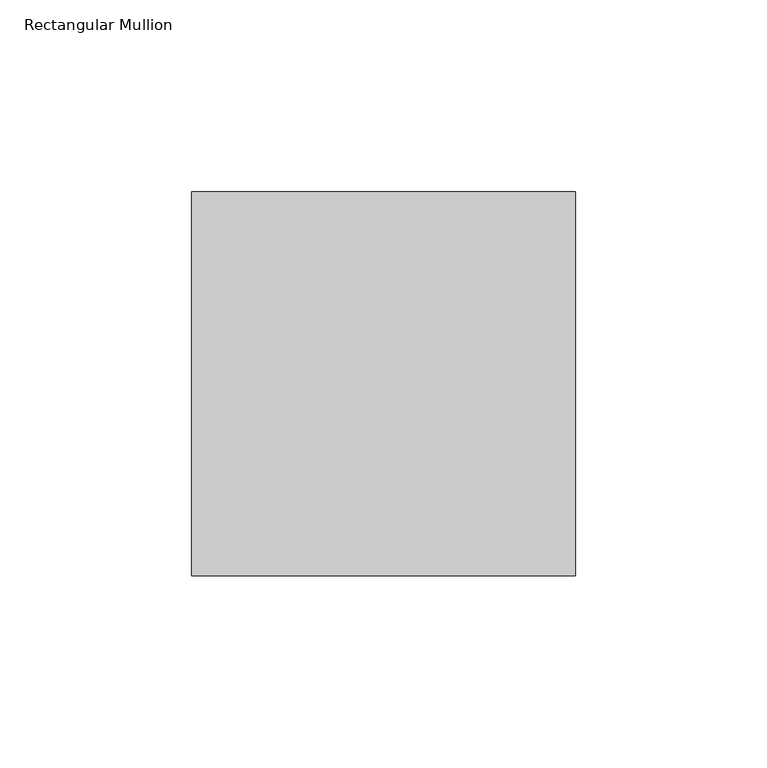
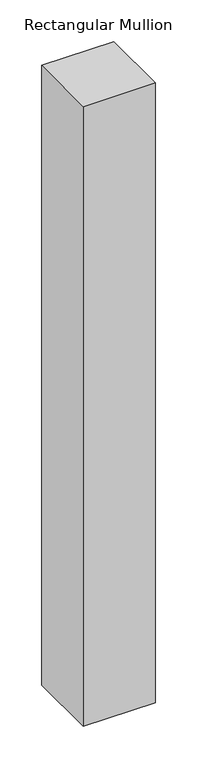
"""IFC4 building model written with IfcOpenShell, lengths in millimetres: member geometry, Rectangular Mullion : 알루미늄_Rectangular Cap_100 x100."""

from ifc_helpers import new_model, si_unit, frame, origin, place, context, project, spatial, polyline, outline, extrude, source, transform, mapped, element, save


def rectangular_mullion_dadccf76(model_context):
    return source(origin(), model_context, "Body", "SweptSolid", [
        extrude(outline(polyline([(0.0, 50.0), (0.0, -50.0), (-100.0, -50.0), (-100.0, 50.0), (0.0, 50.0)])), frame((0.0, 0.0, -910.0), z_axis=(0.0, 0.0, 1.0), x_axis=(1.0, 0.0, 0.0)), (0.0, 0.0, 1.0), 910.0),
    ])


if __name__ == "__main__":
    model = new_model("IFC4")
    model_context = context("Model", 3, world=origin())
    ifc_project = project(units=[si_unit("LENGTHUNIT", "METRE", prefix="MILLI")], contexts=[model_context])
    site = spatial("IfcSite", under=ifc_project)
    building = spatial("IfcBuilding", under=site)
    placement = place(None, origin())
    rectangular_mullion_shape = rectangular_mullion_dadccf76(model_context)
    element("IfcMember", 1, ObjectType="Rectangular Mullion : 알루미늄_Rectangular Cap_100 x100", at=placement, inside=building, context=model_context, shape_type="MappedRepresentation", body=[
        mapped(rectangular_mullion_shape, transform((0.0, 0.0, 0.0), x_axis=(1.0, 0.0, 0.0), y_axis=(0.0, 1.0, 0.0), z_axis=(0.0, 0.0, 1.0))),
    ])
    save(model, "model.ifc")

# Revit data of these elements
# Type "Rectangular Mullion : 알루미늄_Rectangular Cap_100 x100"
#   built-in parameter 1007304 = 0.328084 (stored number, unit not read)
#   built-in parameter 1007301 = 0.164042 (stored number, unit not read)
#   built-in parameter 1007300 = 0.164042 (stored number, unit not read)
# Element 1 (IfcMember, "Rectangular Mullion : 알루미늄_Rectangular Cap_100 x100")
#   Materials on its faces: "00_Metal_Stainless Steel"
# Materials
#   "00_Metal_Stainless Steel": class "Metal", colour RGB 148 148 148, transparency 0, Description = "Steel", Cost = 0
